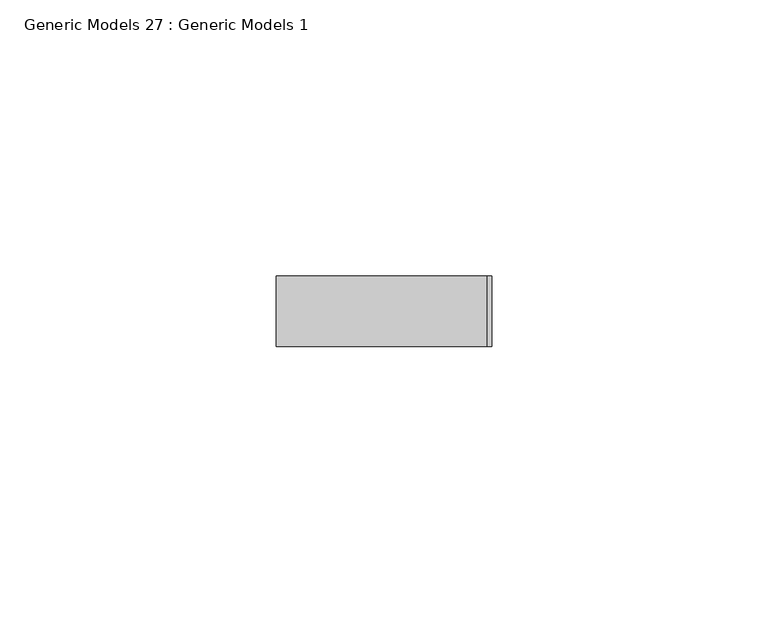
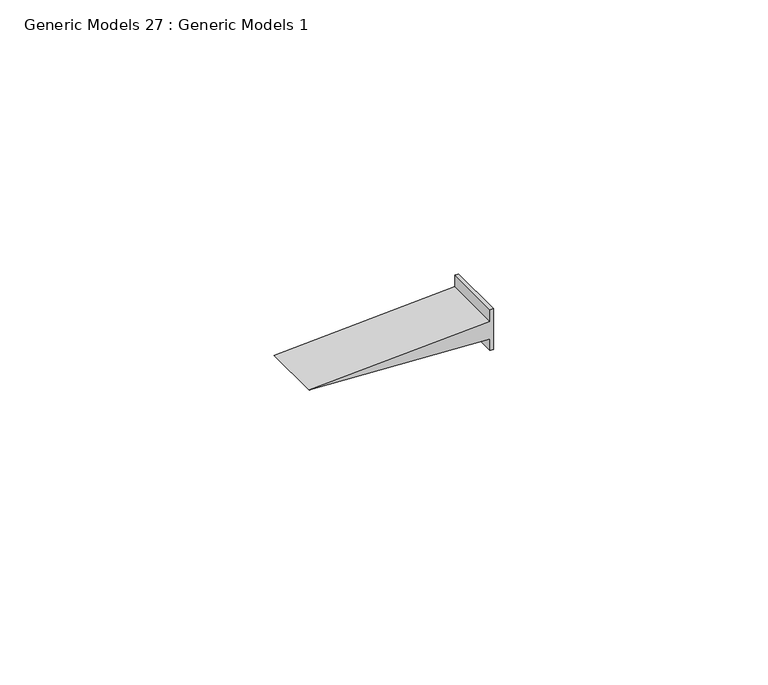
"""IFC4 building model written with IfcOpenShell, lengths in millimetres: proxy geometry, Generic Models 27 : Generic Models 1."""

from ifc_helpers import new_model, si_unit, frame, origin, place, context, project, spatial, polyline, outline, extrude, source, transform, mapped, element, save


def generic_models_27_generic_models_1_58db4025(model_context):
    return source(origin(), model_context, "Body", "SweptSolid", [
        extrude(outline(polyline([(2414.3721662, 49800.66875), (2414.3721662, 49799.875), (2411.8223026, 49799.875), (2409.8255662, 49761.775), (2407.8288298, 49799.875), (2405.2789662, 49799.875), (2405.2789662, 49800.66875), (2414.3721662, 49800.66875)])), frame((0.0, 565.15, 0.0), z_axis=(0.0, 1.0, 0.0), x_axis=(0.0, 0.0, 1.0)), (0.0, 0.0, 1.0), 12.7),
    ])


if __name__ == "__main__":
    model = new_model("IFC4")
    model_context = context("Model", 3, world=origin())
    ifc_project = project(units=[si_unit("LENGTHUNIT", "METRE", prefix="MILLI")], contexts=[model_context])
    site = spatial("IfcSite", under=ifc_project)
    building = spatial("IfcBuilding", under=site)
    placement = place(None, origin())
    generic_models_27_generic_models_1_shape = generic_models_27_generic_models_1_58db4025(model_context)
    element("IfcBuildingElementProxy", 1, Name="Generic Models 27 : Generic Models 1", ObjectType="Generic Models 27 : Generic Models 1", at=placement, inside=building, context=model_context, shape_type="MappedRepresentation", body=[
        mapped(generic_models_27_generic_models_1_shape, transform((0.0, 0.0, 0.0), x_axis=(1.0, 0.0, 0.0), y_axis=(0.0, 1.0, 0.0), z_axis=(0.0, 0.0, 1.0))),
    ])
    save(model, "model.ifc")

# Revit data of these elements
# Element 1 (IfcBuildingElementProxy, "Generic Models 27 : Generic Models 1")
#   Materials on its faces: "ATTACH GYPSUM BOARD TO STUDS AND NOT TO TOP TRACK"
# Materials
#   "ATTACH GYPSUM BOARD TO STUDS AND NOT TO TOP TRACK": class "Generic", colour RGB 48 48 48, transparency 0, Cost = 0
